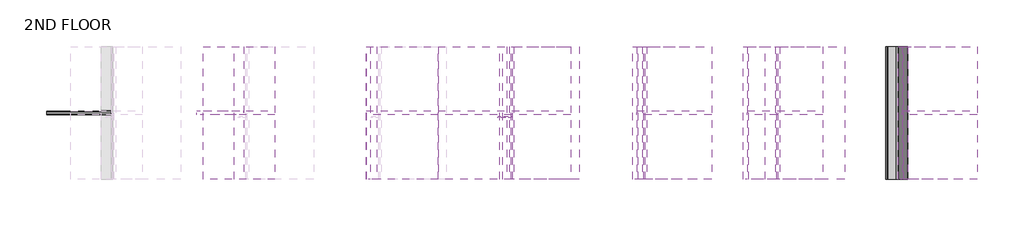
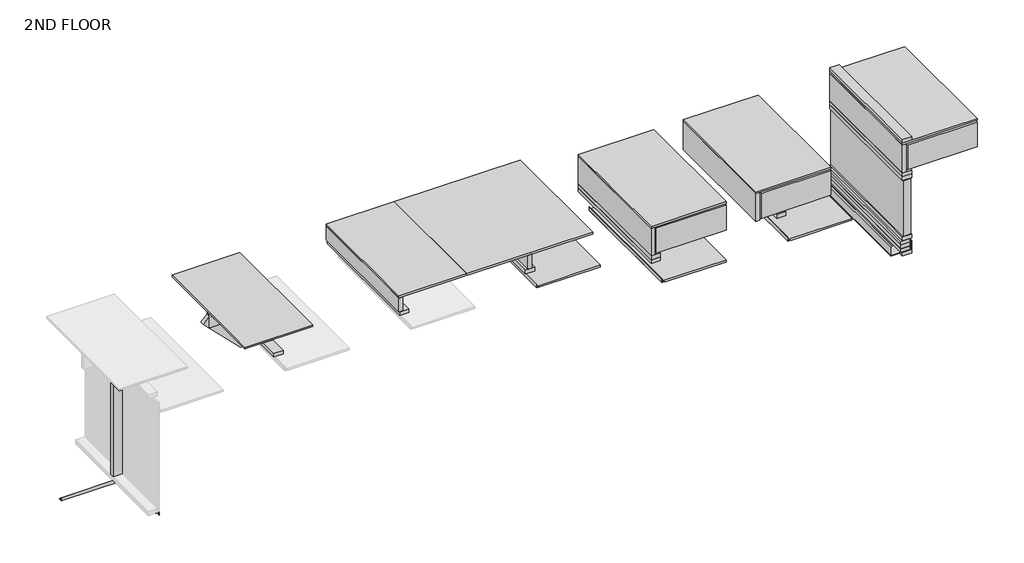
# One storey, part 2 of 2: 51 proxies.
"""IFC4 building model written with IfcOpenShell, lengths in millimetres."""

import ifcopenshell
import ifcopenshell.guid

model = None  # the IFC model being written
_history = None  # IfcOwnerHistory: only IFC2X3 demands one
_inside = {}  # id of a spatial element -> (the spatial element, [elements in it])
_under = {}  # id of a project, library or spatial element -> (it, [spatial elements below it])
_declared = {}  # id of a project -> (the project, [libraries it declares])
_typed = {}  # id of a type object -> (the type object, [elements of that type])
_made_of = {}  # id of a material, layer set ... -> (it, [elements and type objects made of it])


def new_model(schema):
    """Start an empty IFC model of exactly this schema.

    Asked for "IFC4X3", IfcOpenShell would pick the latest addendum, in which some entities
    have other attributes; the version numbers below select the first issue.
    IFC2X3 requires an IfcOwnerHistory on every rooted entity: one is made here for all.
    """
    global model, _history
    if schema == "IFC4X3":
        model = ifcopenshell.file(schema_version=(4, 3, 0, 0))
    else:
        model = ifcopenshell.file(schema=schema)
    _inside.clear()
    _under.clear()
    _declared.clear()
    _typed.clear()
    _made_of.clear()
    _history = None
    if model.schema == "IFC2X3":
        org = make("IfcOrganization", Name="unknown")
        user = make(
            "IfcPersonAndOrganization",
            ThePerson=make("IfcPerson", FamilyName="unknown"),
            TheOrganization=org,
        )
        app = make(
            "IfcApplication",
            ApplicationDeveloper=org,
            Version="unknown",
            ApplicationFullName="unknown",
            ApplicationIdentifier="unknown",
        )
        _history = make(
            "IfcOwnerHistory",
            OwningUser=user,
            OwningApplication=app,
            ChangeAction="ADDED",
            CreationDate=0,
        )
    return model


def make(cls, **values):
    """One entity of the class cls with the attributes given. An attribute that is None is left unset."""
    return model.create_entity(
        cls, **{name: value for name, value in values.items() if value is not None}
    )


def rooted(cls, **values):
    """An entity with a GlobalId (a new one), such as an element, a storey or a relation."""
    return make(cls, GlobalId=ifcopenshell.guid.new(), OwnerHistory=_history, **values)


def si_unit(unit_type, name, prefix=None):
    """IfcSIUnit, for example si_unit("LENGTHUNIT", "METRE", prefix="MILLI")."""
    return make("IfcSIUnit", UnitType=unit_type, Prefix=prefix, Name=name)


def assignment(units):
    """IfcUnitAssignment: the units of a project."""
    return None if units is None else make("IfcUnitAssignment", Units=units)


def point(xyz):
    """IfcCartesianPoint."""
    return None if xyz is None else make("IfcCartesianPoint", Coordinates=xyz)


def direction(xyz):
    """IfcDirection."""
    return None if xyz is None else make("IfcDirection", DirectionRatios=xyz)


def frame(location, z_axis=None, x_axis=None):
    """IfcAxis2Placement3D, a coordinate frame: its origin and axes. An axis left out is left unset."""
    return make(
        "IfcAxis2Placement3D",
        Location=point(location),
        Axis=direction(z_axis),
        RefDirection=direction(x_axis),
    )


def frame_2d(location, x_axis=None):
    """IfcAxis2Placement2D, a coordinate frame in the plane: its origin and x axis."""
    return make(
        "IfcAxis2Placement2D", Location=point(location), RefDirection=direction(x_axis)
    )


def origin():
    """The frame at (0, 0, 0) with its axes left unset."""
    return frame((0.0, 0.0, 0.0))


def place(relative_to, where):
    """IfcLocalPlacement: puts the frame where relative to a parent placement (None: the world)."""
    return make(
        "IfcLocalPlacement", PlacementRelTo=relative_to, RelativePlacement=where
    )


def context(
    kind, dimensions, precision=None, world=None, true_north=None, identifier=None
):
    """IfcGeometricRepresentationContext, for example the 3D "Model" context."""
    return make(
        "IfcGeometricRepresentationContext",
        ContextIdentifier=identifier,
        ContextType=kind,
        CoordinateSpaceDimension=dimensions,
        Precision=precision,
        WorldCoordinateSystem=world,
        TrueNorth=true_north,
    )


def project(units=None, contexts=None):
    """IfcProject with its units and contexts."""
    return rooted(
        "IfcProject",
        Name="project",
        RepresentationContexts=contexts,
        UnitsInContext=assignment(units),
    )


def spatial(cls, under=None, at=None, **own):
    """A site, building, storey or space (cls), placed at a placement, below another one or the project."""
    s = rooted(cls, ObjectPlacement=at, **own)
    if under is not None:
        _under.setdefault(under.id(), (under, []))[1].append(s)
    return s


def polyline(points):
    """IfcPolyline through the points."""
    return make("IfcPolyline", Points=[point(p) for p in points])


def circle_curve(where, radius):
    """IfcCircle in the frame where."""
    return make("IfcCircle", Position=where, Radius=radius)


def trimmed(basis, trim1, trim2, sense, master):
    """IfcTrimmedCurve: the piece of a basis curve between two trims."""
    return make(
        "IfcTrimmedCurve",
        BasisCurve=basis,
        Trim1=trim1,
        Trim2=trim2,
        SenseAgreement=sense,
        MasterRepresentation=master,
    )


def segment(curve, same_sense, transition):
    """IfcCompositeCurveSegment."""
    return make(
        "IfcCompositeCurveSegment",
        Transition=transition,
        SameSense=same_sense,
        ParentCurve=curve,
    )


def composite_curve(segments, self_intersect=None):
    """IfcCompositeCurve: segments joined end to end."""
    return make("IfcCompositeCurve", Segments=segments, SelfIntersect=self_intersect)


def outline(outer, holes=None, kind="AREA"):
    """IfcArbitraryClosedProfileDef: a profile drawn as a closed curve; with holes, ...WithVoids."""
    if holes is None:
        return make("IfcArbitraryClosedProfileDef", ProfileType=kind, OuterCurve=outer)
    return make(
        "IfcArbitraryProfileDefWithVoids",
        ProfileType=kind,
        OuterCurve=outer,
        InnerCurves=holes,
    )


def extrude(swept, where, along, depth):
    """IfcExtrudedAreaSolid: the profile swept, set in the frame where, extruded along a direction by depth."""
    return make(
        "IfcExtrudedAreaSolid",
        SweptArea=swept,
        Position=where,
        ExtrudedDirection=direction(along),
        Depth=depth,
    )


def shape(context_of_items, identifier, shape_type, items):
    """IfcShapeRepresentation: the items that make up one representation, for example the "Body"."""
    return make(
        "IfcShapeRepresentation",
        ContextOfItems=context_of_items,
        RepresentationIdentifier=identifier,
        RepresentationType=shape_type,
        Items=items,
    )


def source(mapping_origin, context_of_items, identifier, shape_type, items):
    """IfcRepresentationMap: a shape defined once, which mapped items show again and again."""
    return make(
        "IfcRepresentationMap",
        MappingOrigin=mapping_origin,
        MappedRepresentation=shape(context_of_items, identifier, shape_type, items),
    )


def transform(
    local_origin,
    x_axis=None,
    y_axis=None,
    z_axis=None,
    scale=None,
    scale2=None,
    scale3=None,
    uniform=True,
):
    """IfcCartesianTransformationOperator3D, or its non-uniform kind. x_axis, y_axis, z_axis: its Axis1, 2, 3."""
    if uniform:
        return make(
            "IfcCartesianTransformationOperator3D",
            Axis1=direction(x_axis),
            Axis2=direction(y_axis),
            LocalOrigin=point(local_origin),
            Scale=scale,
            Axis3=direction(z_axis),
        )
    return make(
        "IfcCartesianTransformationOperator3DnonUniform",
        Axis1=direction(x_axis),
        Axis2=direction(y_axis),
        LocalOrigin=point(local_origin),
        Scale=scale,
        Axis3=direction(z_axis),
        Scale2=scale2,
        Scale3=scale3,
    )


def mapped(mapping_source, mapping_target):
    """IfcMappedItem: shows the shape of a source again, moved by a transform."""
    return make(
        "IfcMappedItem", MappingSource=mapping_source, MappingTarget=mapping_target
    )


def made_of(thing, what):
    """Note that an element or type object is made of a material, layer set ...; save() writes the relation."""
    if what is not None:
        _made_of.setdefault(what.id(), (what, []))[1].append(thing)
    return thing


def element(
    cls,
    number,
    at=None,
    inside=None,
    cuts=None,
    type_object=None,
    material=None,
    context=None,
    identifier="Body",
    shape_type=None,
    held_by="IfcProductDefinitionShape",
    body=None,
    shapes=None,
    **own,
):
    """One element of the class cls, such as IfcWall. Its Tag is "e" and its number.

    at: its placement. inside: the storey or other place that contains it. cuts: it is an
    opening in that element (IfcRelVoidsElement). A single representation is given by context,
    identifier, shape_type and body (its items); several are given by shapes. held_by: the class
    of the entity that holds the representations. save() writes the other relations.
    """
    e = rooted(cls, Tag="e%d" % number, ObjectPlacement=at, **own)
    if body is not None:
        shapes = [shape(context, identifier, shape_type, body)]
    if shapes is not None:
        e.Representation = make(held_by, Representations=shapes)
    if inside is not None:
        _inside.setdefault(inside.id(), (inside, []))[1].append(e)
    if cuts is not None:
        rooted(
            "IfcRelVoidsElement", RelatingBuildingElement=cuts, RelatedOpeningElement=e
        )
    if type_object is not None:
        _typed.setdefault(type_object.id(), (type_object, []))[1].append(e)
    return made_of(e, material)


def aggregate(whole, parts):
    """IfcRelAggregates: a whole, such as a stair, and the parts it consists of."""
    return rooted("IfcRelAggregates", RelatingObject=whole, RelatedObjects=parts)


def save(model, path):
    """Write the relations noted so far, then the file.

    IfcRelAggregates (storeys below a building ...), IfcRelContainedInSpatialStructure (elements
    in a storey), IfcRelDefinesByType, IfcRelAssociatesMaterial and IfcRelDeclares: one each for
    every whole, place, type object, material and project.
    """
    for whole, parts in _under.values():
        aggregate(whole, parts)
    for where, things in _inside.values():
        rooted(
            "IfcRelContainedInSpatialStructure",
            RelatedElements=things,
            RelatingStructure=where,
        )
    for kind, things in _typed.values():
        rooted("IfcRelDefinesByType", RelatedObjects=things, RelatingType=kind)
    for what, things in _made_of.values():
        rooted("IfcRelAssociatesMaterial", RelatedObjects=things, RelatingMaterial=what)
    for by, libraries in _declared.values():
        rooted("IfcRelDeclares", RelatingContext=by, RelatedDefinitions=libraries)
    model.write(path)


def generic_models_10_generic_models_1_ea081297(model_context):
    return source(origin(), model_context, "Body", "SweptSolid", [
        extrude(outline(polyline([(49758.6, 0.0), (49720.5, 0.0), (49720.5, 1219.2), (49758.6, 1219.2), (49758.6, 0.0)])), frame((0.0, 0.0, 5507.83125), z_axis=(0.0, 0.0, 1.0), x_axis=(1.0, 0.0, 0.0)), (0.0, 0.0, 1.0), 139.7),
    ])


def generic_models_102_generic_models_1_8a2dd616(model_context):
    return source(origin(), model_context, "Body", "SweptSolid", [
        extrude(outline(composite_curve([segment(polyline([(4498.578125, 52222.4), (4510.823229, 52207.8068534), (4508.6950617, 52206.021109), (4497.282664, 52219.621875), (4414.3677682, 52219.621875)]), True, "CONTINUOUS"), segment(trimmed(circle_curve(frame_2d((4414.4412941, 52217.6381931)), 1.9850441), [point((4414.3677682, 52219.621875))], [point((4412.45625, 52217.6381931))], True, "CARTESIAN"), True, "CONTINUOUS"), segment(polyline([(4412.45625, 52217.6381931), (4412.45625, 52023.9610661)]), True, "CONTINUOUS"), segment(trimmed(circle_curve(frame_2d((4414.4419899, 52023.9610661)), 1.9857399), [point((4412.45625, 52023.9610661))], [point((4414.3365981, 52021.978125))], True, "CARTESIAN"), True, "CONTINUOUS"), segment(polyline([(4414.3365981, 52021.978125), (4497.282664, 52021.978125), (4508.718285, 52035.6065673), (4510.8464522, 52033.820823), (4498.578125, 52019.2), (4414.440625, 52019.2)]), True, "CONTINUOUS"), segment(trimmed(circle_curve(frame_2d((4414.440625, 52023.9625)), 4.7625), [point((4414.440625, 52019.2))], [point((4409.678125, 52023.9625))], False, "CARTESIAN"), True, "CONTINUOUS"), segment(polyline([(4409.678125, 52023.9625), (4409.678125, 52217.6375)]), True, "CONTINUOUS"), segment(trimmed(circle_curve(frame_2d((4414.440625, 52217.6375)), 4.7625), [point((4409.678125, 52217.6375))], [point((4414.440625, 52222.4))], False, "CARTESIAN"), True, "CONTINUOUS"), segment(polyline([(4414.440625, 52222.4), (4498.578125, 52222.4)]), True, "CONTINUOUS")], self_intersect=False)), frame((0.0, 0.0, 0.0), z_axis=(0.0, 1.0, 0.0), x_axis=(0.0, 0.0, 1.0)), (0.0, 0.0, 1.0), 1219.2),
    ])


def generic_models_103_generic_models_1_250a6a11(model_context):
    return source(origin(), model_context, "Body", "SweptSolid", [
        extrude(outline(polyline([(49784.0, 0.0), (49695.1, 0.0), (49695.1, 1219.2), (49784.0, 1219.2), (49784.0, 0.0)])), frame((0.0, 0.0, 5264.15), z_axis=(0.0, 0.0, 1.0), x_axis=(1.0, 0.0, 0.0)), (0.0, 0.0, 1.0), 38.1),
    ])


def generic_models_104_generic_models_1_af33e5d9(model_context):
    return source(origin(), model_context, "Body", "SweptSolid", [
        extrude(outline(polyline([(52206.021109, 0.0), (52117.121109, 0.0), (52117.121109, 1219.2), (52206.021109, 1219.2), (52206.021109, 0.0)])), frame((0.0, 0.0, 4412.45625), z_axis=(0.0, 0.0, 1.0), x_axis=(1.0, 0.0, 0.0)), (0.0, 0.0, 1.0), 38.1),
    ])


def generic_models_108_generic_models_1_496acf5e(model_context):
    return source(origin(), model_context, "Body", "SweptSolid", [
        extrude(outline(polyline([(52216.05, 1219.2), (52216.05, 0.0), (52139.85, 0.0), (52139.85, 1219.2), (52216.05, 1219.2)])), frame((0.0, 0.0, 4570.4125), z_axis=(0.0, 0.0, 1.0), x_axis=(1.0, 0.0, 0.0)), (0.0, 0.0, 1.0), 565.15),
    ])


def generic_models_109_generic_models_1_8619d77b(model_context):
    return source(origin(), model_context, "Body", "SweptSolid", [
        extrude(outline(polyline([(51003.2, 0.0), (50914.3, 0.0), (50914.3, 1219.2), (51003.2, 1219.2), (51003.2, 0.0)])), frame((0.0, 0.0, 5184.378125), z_axis=(0.0, 0.0, 1.0), x_axis=(1.0, 0.0, 0.0)), (0.0, 0.0, 1.0), 38.1),
    ])


def generic_models_110_generic_models_1_6bdce9b6(model_context):
    return source(origin(), model_context, "Body", "SweptSolid", [
        extrude(outline(polyline([(51642.1451407, 1219.2), (51642.1451407, 0.0), (50914.3, 0.0), (50914.3, 1219.2), (51642.1451407, 1219.2)])), frame((0.0, 0.0, 5508.228125), z_axis=(0.0, 0.0, 1.0), x_axis=(1.0, 0.0, 0.0)), (0.0, 0.0, 1.0), 19.05),
    ])


def generic_models_112_generic_models_65_d168d7b0(model_context):
    return source(origin(), model_context, "Body", "SweptSolid", [
        extrude(outline(polyline([(50952.4, 592.1375), (50952.4, 630.2375), (51642.1451407, 630.2375), (51642.1451407, 592.1375), (50952.4, 592.1375)])), frame((0.0, 0.0, 5222.478125), z_axis=(0.0, 0.0, 1.0), x_axis=(1.0, 0.0, 0.0)), (0.0, 0.0, 1.0), 285.75),
    ])


def generic_models_113_generic_models_1_101608ab(model_context):
    return source(origin(), model_context, "Body", "SweptSolid", [
        extrude(outline(polyline([(52171.6, 0.0), (52133.5, 0.0), (52133.5, 1219.2), (52171.6, 1219.2), (52171.6, 0.0)])), frame((0.0, 0.0, 5222.478125), z_axis=(0.0, 0.0, 1.0), x_axis=(1.0, 0.0, 0.0)), (0.0, 0.0, 1.0), 285.75),
    ])


def generic_models_114_generic_models_1_a6fb1c2c(model_context):
    return source(origin(), model_context, "Body", "SweptSolid", [
        extrude(outline(polyline([(51642.1451407, 1219.2), (51642.1451407, 0.0), (50965.9242022, 0.0), (50965.9242022, 1219.2), (51642.1451407, 1219.2)])), frame((0.0, 0.0, 5237.6235034), z_axis=(0.0, 0.0, 1.0), x_axis=(1.0, 0.0, 0.0)), (0.0, 0.0, 1.0), 254.0),
    ])


def generic_models_12_generic_models_46_b8a9a4e8(model_context):
    return source(origin(), model_context, "Body", "SweptSolid", [
        extrude(outline(polyline([(49757.8505137, 0.0), (49721.1284797, 0.0), (49721.1284797, 1219.2), (49757.8505137, 1219.2), (49757.8505137, 0.0)])), frame((0.0, 0.0, 5505.7509163), z_axis=(0.0, 0.0, 1.0), x_axis=(1.0, 0.0, 0.0)), (0.0, 0.0, 1.0), 1.5875),
    ])


def generic_models_13_generic_models_65_9e643fb9(model_context):
    return source(origin(), model_context, "Body", "SweptSolid", [
        extrude(outline(polyline([(49128.3625, 592.1375), (49128.3625, 630.2375), (50347.5625, 630.2375), (50347.5625, 592.1375), (49128.3625, 592.1375)])), frame((0.0, 0.0, 5507.83125), z_axis=(0.0, 0.0, 1.0), x_axis=(1.0, 0.0, 0.0)), (0.0, 0.0, 1.0), 139.7),
    ])


def generic_models_14_generic_models_1_e8c90d4c(model_context):
    return source(origin(), model_context, "Body", "SweptSolid", [
        extrude(outline(polyline([(2277.1204978, 49799.875), (2239.0204978, 49799.875), (2239.0204978, 49825.275), (2240.6079978, 49825.275), (2240.6079978, 49801.4625), (2277.1204978, 49801.4625), (2277.1204978, 49799.875)])), frame((0.0, 0.0, 0.0), z_axis=(0.0, 1.0, 0.0), x_axis=(0.0, 0.0, 1.0)), (0.0, 0.0, 1.0), 1219.2),
    ])


def generic_models_22_generic_models_1_e5767157(model_context):
    return source(origin(), model_context, "Body", "SweptSolid", [
        extrude(outline(polyline([(2409.6091, 49800.66875), (2409.6091, 49799.875), (2407.0592364, 49799.875), (2405.4618473, 49749.075), (2404.6631527, 49749.075), (2403.0657636, 49799.875), (2400.5159, 49799.875), (2400.5159, 49800.66875), (2409.6091, 49800.66875)])), frame((0.0, 565.15, 0.0), z_axis=(0.0, 1.0, 0.0), x_axis=(0.0, 0.0, 1.0)), (0.0, 0.0, 1.0), 12.7),
    ])


def generic_models_228_generic_models_1_053e8907(model_context):
    return source(origin(), model_context, "Body", "SweptSolid", [
        extrude(outline(composite_curve([segment(polyline([(592.1375, 4235.45), (592.1375, 4267.2)]), True, "CONTINUOUS"), segment(trimmed(circle_curve(frame_2d((592.1375, 4264.025)), 3.175), [point((592.1375, 4267.2))], [point((595.3125, 4264.025))], False, "CARTESIAN"), True, "CONTINUOUS"), segment(polyline([(595.3125, 4264.025), (595.3125, 4240.2125)]), True, "CONTINUOUS"), segment(trimmed(circle_curve(frame_2d((596.9, 4240.2125)), 1.5875), [point((595.3125, 4240.2125))], [point((596.9, 4238.625))], True, "CARTESIAN"), True, "CONTINUOUS"), segment(polyline([(596.9, 4238.625), (620.7125, 4238.625)]), True, "CONTINUOUS"), segment(trimmed(circle_curve(frame_2d((620.7125, 4235.45)), 3.175), [point((620.7125, 4238.625))], [point((623.8875, 4235.45))], False, "CARTESIAN"), True, "CONTINUOUS"), segment(polyline([(623.8875, 4235.45), (592.1375, 4235.45)]), True, "CONTINUOUS")], self_intersect=False)), frame((46753.4625, 0.0, 0.0), z_axis=(1.0, 0.0, 0.0), x_axis=(0.0, 1.0, 0.0)), (0.0, 0.0, 1.0), 609.6),
    ])


def generic_models_233_generic_models_1_ae5bae41(model_context):
    return source(origin(), model_context, "Body", "SweptSolid", [
        extrude(outline(polyline([(48564.8, 0.0), (48475.9, 0.0), (48475.9, 1219.2), (48564.8, 1219.2), (48564.8, 0.0)])), frame((0.0, 0.0, 5467.35), z_axis=(0.0, 0.0, 1.0), x_axis=(1.0, 0.0, 0.0)), (0.0, 0.0, 1.0), 38.1),
    ])


def generic_models_236_generic_models_1_f8917e71(model_context):
    return source(origin(), model_context, "Body", "SweptSolid", [
        extrude(outline(polyline([(48507.65, 0.0), (48469.55, 0.0), (48469.55, 1219.2), (48507.65, 1219.2), (48507.65, 0.0)])), frame((0.0, 0.0, 5507.83125), z_axis=(0.0, 0.0, 1.0), x_axis=(1.0, 0.0, 0.0)), (0.0, 0.0, 1.0), 139.7),
    ])


def generic_models_237_generic_models_65_1df05f16(model_context):
    return source(origin(), model_context, "Body", "SweptSolid", [
        extrude(outline(polyline([(48469.55, 592.1375), (48469.55, 630.2375), (49128.3625, 630.2375), (49128.3625, 592.1375), (48469.55, 592.1375)])), frame((0.0, 0.0, 5507.83125), z_axis=(0.0, 0.0, 1.0), x_axis=(1.0, 0.0, 0.0)), (0.0, 0.0, 1.0), 139.7),
    ])


def generic_models_240_generic_models_1_611786cf(model_context):
    return source(origin(), model_context, "Body", "SweptSolid", [
        extrude(outline(polyline([(49128.3625, 1219.2), (49128.3625, 0.0), (48469.55, 0.0), (48469.55, 1219.2), (49128.3625, 1219.2)])), frame((0.0, 0.0, 5649.9125), z_axis=(0.0, 0.0, 1.0), x_axis=(1.0, 0.0, 0.0)), (0.0, 0.0, 1.0), 19.05),
    ])


def generic_models_246_generic_models_1_33f707d8(model_context):
    return source(origin(), model_context, "Body", "SweptSolid", [
        extrude(outline(composite_curve([segment(polyline([(4267.2, 47363.0625), (4267.2, 47331.3125)]), True, "CONTINUOUS"), segment(trimmed(circle_curve(frame_2d((4267.2, 47334.4875)), 3.175), [point((4267.2, 47331.3125))], [point((4264.025, 47334.4875))], False, "CARTESIAN"), True, "CONTINUOUS"), segment(polyline([(4264.025, 47334.4875), (4264.025, 47358.3)]), True, "CONTINUOUS"), segment(trimmed(circle_curve(frame_2d((4262.4375, 47358.3)), 1.5875), [point((4264.025, 47358.3))], [point((4262.4375, 47359.8875))], True, "CARTESIAN"), True, "CONTINUOUS"), segment(polyline([(4262.4375, 47359.8875), (4238.625, 47359.8875)]), True, "CONTINUOUS"), segment(trimmed(circle_curve(frame_2d((4238.625, 47363.0625)), 3.175), [point((4238.625, 47359.8875))], [point((4235.45, 47363.0625))], False, "CARTESIAN"), True, "CONTINUOUS"), segment(polyline([(4235.45, 47363.0625), (4267.2, 47363.0625)]), True, "CONTINUOUS")], self_intersect=False)), frame((0.0, 0.0, 0.0), z_axis=(0.0, 1.0, 0.0), x_axis=(0.0, 0.0, 1.0)), (0.0, 0.0, 1.0), 1219.2),
    ])


def generic_models_248_generic_models_65_f6c484d7(model_context):
    return source(origin(), model_context, "Body", "SweptSolid", [
        extrude(outline(polyline([(47345.6, 592.1375), (47256.7, 592.1375), (47256.7, 630.2375), (47345.6, 630.2375), (47345.6, 592.1375)])), frame((0.0, 0.0, 4305.3), z_axis=(0.0, 0.0, 1.0), x_axis=(1.0, 0.0, 0.0)), (0.0, 0.0, 1.0), 1162.05),
    ])


def generic_models_267_generic_models_65_11354230(model_context):
    return source(origin(), model_context, "Body", "SweptSolid", [
        extrude(outline(polyline([(0.0, -38.1), (0.0, 0.0), (514.35, 0.0), (514.35, -38.1), (0.0, -38.1)])), frame((47276.4596037, 592.1375, 5202.484661), z_axis=(0.7071067811865633, 0.0, 0.7071067811865317), x_axis=(-0.7071067811865317, 0.0, 0.7071067811865633)), (0.0, 0.0, 1.0), 88.9),
    ])


def generic_models_29_generic_models_1_59087225(model_context):
    return source(origin(), model_context, "Body", "SweptSolid", [
        extrude(outline(polyline([(50347.5625, 1219.2), (50347.5625, 0.0), (49128.3625, 0.0), (49128.3625, 1219.2), (50347.5625, 1219.2)])), frame((0.0, 0.0, 5647.53125), z_axis=(0.0, 0.0, 1.0), x_axis=(1.0, 0.0, 0.0)), (0.0, 0.0, 1.0), 19.05),
    ])


def generic_models_226_generic_models_1_7dc37832(model_context):
    return source(origin(), model_context, "Body", "SweptSolid", [
        extrude(outline(polyline([(5263.35625, 49733.4159), (5263.35625, 49742.5091), (5264.15, 49742.5091), (5264.15, 49739.9592364), (5314.95, 49738.3618473), (5314.95, 49737.5631527), (5264.15, 49735.9657636), (5264.15, 49733.4159), (5263.35625, 49733.4159)])), frame((0.0, 565.15, 0.0), z_axis=(0.0, 1.0, 0.0), x_axis=(0.0, 0.0, 1.0)), (0.0, 0.0, 1.0), 12.7),
    ])


def generic_models_37_generic_models_1_916dd7c6(model_context):
    return source(origin(), model_context, "Body", "SweptSolid", [
        extrude(outline(polyline([(2409.6091, 49675.25625), (2400.5159, 49675.25625), (2400.5159, 49676.05), (2403.0657636, 49676.05), (2404.6631527, 49726.85), (2405.4618473, 49726.85), (2407.0592364, 49676.05), (2409.6091, 49676.05), (2409.6091, 49675.25625)])), frame((0.0, 565.15, 0.0), z_axis=(0.0, 1.0, 0.0), x_axis=(0.0, 0.0, 1.0)), (0.0, 0.0, 1.0), 12.7),
    ])


def generic_models_202_generic_models_1_0ad20a8b(model_context):
    return source(origin(), model_context, "Body", "SweptSolid", [
        extrude(outline(polyline([(2253.330428, 49813.3451407), (2242.217928, 49813.3451407), (2242.217928, 49826.0451407), (2234.280428, 49828.9341545), (2234.280428, 50422.9451407), (2253.330428, 50422.9451407), (2253.330428, 49813.3451407)])), frame((0.0, 0.0, 0.0), z_axis=(0.0, 1.0, 0.0), x_axis=(0.0, 0.0, 1.0)), (0.0, 0.0, 1.0), 1219.2),
    ])


def generic_models_71_generic_models_1_508a995f(model_context):
    return source(origin(), model_context, "Body", "SweptSolid", [
        extrude(outline(polyline([(50952.4, 0.0), (50914.3, 0.0), (50914.3, 1219.2), (50952.4, 1219.2), (50952.4, 0.0)])), frame((0.0, 0.0, 5222.478125), z_axis=(0.0, 0.0, 1.0), x_axis=(1.0, 0.0, 0.0)), (0.0, 0.0, 1.0), 285.75),
    ])


def generic_models_87_generic_models_1_55a64953(model_context):
    return source(origin(), model_context, "Body", "SweptSolid", [
        extrude(outline(polyline([(51968.4, 0.0), (51930.3, 0.0), (51930.3, 1219.2), (51968.4, 1219.2), (51968.4, 0.0)])), frame((0.0, 0.0, 5222.478125), z_axis=(0.0, 0.0, 1.0), x_axis=(1.0, 0.0, 0.0)), (0.0, 0.0, 1.0), 285.75),
    ])


model = new_model("IFC4")

# Units and contexts
model_context = context("Model", 3, world=origin())
ifc_project = project(units=[si_unit("LENGTHUNIT", "METRE", prefix="MILLI")], contexts=[model_context])

# Site, building, storey
site = spatial("IfcSite", under=ifc_project)
building = spatial("IfcBuilding", under=site)
storey = spatial("IfcBuildingStorey", under=building, Name="2ND FLOOR", Elevation=3657.6)

# Proxies
placement = place(None, origin())
generic_models_10_generic_models_1_shape = generic_models_10_generic_models_1_ea081297(model_context)
element("IfcBuildingElementProxy", 1, Name="Generic Models 10 : Generic Models 1", ObjectType="Generic Models 10 : Generic Models 1", at=placement, inside=storey, context=model_context, shape_type="MappedRepresentation", body=[
    mapped(generic_models_10_generic_models_1_shape, transform((0.0, 0.0, 0.0), x_axis=(1.0, 0.0, 0.0), y_axis=(0.0, 1.0, 0.0), z_axis=(0.0, 0.0, 1.0))),
])
generic_models_102_generic_models_1_shape = generic_models_102_generic_models_1_8a2dd616(model_context)
element("IfcBuildingElementProxy", 2, Name="Generic Models 102 : Generic Models 1", ObjectType="Generic Models 102 : Generic Models 1", at=placement, inside=storey, context=model_context, shape_type="MappedRepresentation", body=[
    mapped(generic_models_102_generic_models_1_shape, transform((1219.2, 0.0, 0.0), x_axis=(1.0, 0.0, 0.0), y_axis=(0.0, 1.0, 0.0), z_axis=(0.0, 0.0, 1.0))),
])
generic_models_103_generic_models_1_shape = generic_models_103_generic_models_1_250a6a11(model_context)
element("IfcBuildingElementProxy", 3, Name="Generic Models 103 : Generic Models 1", ObjectType="Generic Models 103 : Generic Models 1", at=placement, inside=storey, context=model_context, shape_type="MappedRepresentation", body=[
    mapped(generic_models_103_generic_models_1_shape, transform((3657.6, 0.0, -892.571875), x_axis=(1.0, 0.0, 0.0), y_axis=(0.0, 1.0, 0.0), z_axis=(0.0, 0.0, 1.0))),
])
generic_models_104_generic_models_1_shape = generic_models_104_generic_models_1_af33e5d9(model_context)
element("IfcBuildingElementProxy", 4, Name="Generic Models 104 : Generic Models 1", ObjectType="Generic Models 104 : Generic Models 1", at=placement, inside=storey, context=model_context, shape_type="MappedRepresentation", body=[
    mapped(generic_models_104_generic_models_1_shape, transform((1219.2, 0.0, 0.0), x_axis=(1.0, 0.0, 0.0), y_axis=(0.0, 1.0, 0.0), z_axis=(0.0, 0.0, 1.0))),
])
element("IfcBuildingElementProxy", 5, Name="Generic Models 105 : Generic Models 1", ObjectType="Generic Models 105 : Generic Models 1", at=placement, inside=storey, context=model_context, shape_type="MappedRepresentation", body=[
    mapped(generic_models_103_generic_models_1_shape, transform((3641.221109, 0.0, -813.59375), x_axis=(1.0, 0.0, 0.0), y_axis=(0.0, 1.0, 0.0), z_axis=(0.0, 0.0, 1.0))),
])
element("IfcBuildingElementProxy", 6, Name="Generic Models 106 : Generic Models 1", ObjectType="Generic Models 106 : Generic Models 1", at=placement, inside=storey, context=model_context, shape_type="MappedRepresentation", body=[
    mapped(generic_models_103_generic_models_1_shape, transform((3641.221109, 0.0, -775.49375), x_axis=(1.0, 0.0, 0.0), y_axis=(0.0, 1.0, 0.0), z_axis=(0.0, 0.0, 1.0))),
])
element("IfcBuildingElementProxy", 7, Name="Generic Models 107 : Generic Models 1", ObjectType="Generic Models 107 : Generic Models 1", at=placement, inside=storey, context=model_context, shape_type="MappedRepresentation", body=[
    mapped(generic_models_103_generic_models_1_shape, transform((3657.6, 0.0, -737.39375), x_axis=(1.0, 0.0, 0.0), y_axis=(0.0, 1.0, 0.0), z_axis=(0.0, 0.0, 1.0))),
])
generic_models_108_generic_models_1_shape = generic_models_108_generic_models_1_496acf5e(model_context)
element("IfcBuildingElementProxy", 8, Name="Generic Models 108 : Generic Models 1", ObjectType="Generic Models 108 : Generic Models 1", at=placement, inside=storey, context=model_context, shape_type="MappedRepresentation", body=[
    mapped(generic_models_108_generic_models_1_shape, transform((1219.2, 0.0, 0.0), x_axis=(1.0, 0.0, 0.0), y_axis=(0.0, 1.0, 0.0), z_axis=(0.0, 0.0, 1.0))),
])
generic_models_109_generic_models_1_shape = generic_models_109_generic_models_1_8619d77b(model_context)
element("IfcBuildingElementProxy", 9, Name="Generic Models 109 : Generic Models 1", ObjectType="Generic Models 109 : Generic Models 1", at=placement, inside=storey, context=model_context, shape_type="MappedRepresentation", body=[
    mapped(generic_models_109_generic_models_1_shape, transform((2438.4, 0.0, 0.0), x_axis=(1.0, 0.0, 0.0), y_axis=(0.0, 1.0, 0.0), z_axis=(0.0, 0.0, 1.0))),
])
generic_models_110_generic_models_1_shape = generic_models_110_generic_models_1_6bdce9b6(model_context)
element("IfcBuildingElementProxy", 10, Name="Generic Models 110 : Generic Models 1", ObjectType="Generic Models 110 : Generic Models 1", at=placement, inside=storey, context=model_context, shape_type="MappedRepresentation", body=[
    mapped(generic_models_110_generic_models_1_shape, transform((2438.4, 0.0, 0.0), x_axis=(1.0, 0.0, 0.0), y_axis=(0.0, 1.0, 0.0), z_axis=(0.0, 0.0, 1.0))),
])
element("IfcBuildingElementProxy", 11, Name="Generic Models 111 : Generic Models 1", ObjectType="Generic Models 111 : Generic Models 1", at=placement, inside=storey, context=model_context, shape_type="MappedRepresentation", body=[
    mapped(generic_models_109_generic_models_1_shape, transform((2438.4, 0.0, -38.1), x_axis=(1.0, 0.0, 0.0), y_axis=(0.0, 1.0, 0.0), z_axis=(0.0, 0.0, 1.0))),
])
generic_models_112_generic_models_65_shape = generic_models_112_generic_models_65_d168d7b0(model_context)
element("IfcBuildingElementProxy", 12, Name="Generic Models 112 : Generic Models 65", ObjectType="Generic Models 112 : Generic Models 65", at=placement, inside=storey, context=model_context, shape_type="MappedRepresentation", body=[
    mapped(generic_models_112_generic_models_65_shape, transform((2438.4, 0.0, 0.0), x_axis=(1.0, 0.0, 0.0), y_axis=(0.0, 1.0, 0.0), z_axis=(0.0, 0.0, 1.0))),
])
generic_models_113_generic_models_1_shape = generic_models_113_generic_models_1_101608ab(model_context)
element("IfcBuildingElementProxy", 13, Name="Generic Models 113 : Generic Models 1", ObjectType="Generic Models 113 : Generic Models 1", at=placement, inside=storey, context=model_context, shape_type="MappedRepresentation", body=[
    mapped(generic_models_113_generic_models_1_shape, transform((1219.2, 0.0, 0.0), x_axis=(1.0, 0.0, 0.0), y_axis=(0.0, 1.0, 0.0), z_axis=(0.0, 0.0, 1.0))),
])
generic_models_114_generic_models_1_shape = generic_models_114_generic_models_1_a6fb1c2c(model_context)
element("IfcBuildingElementProxy", 14, Name="Generic Models 114 : Generic Models 1", ObjectType="Generic Models 114 : Generic Models 1", at=placement, inside=storey, context=model_context, shape_type="MappedRepresentation", body=[
    mapped(generic_models_114_generic_models_1_shape, transform((2438.4, 0.0, 0.0), x_axis=(1.0, 0.0, 0.0), y_axis=(0.0, 1.0, 0.0), z_axis=(0.0, 0.0, 1.0))),
])
element("IfcBuildingElementProxy", 15, Name="Generic Models 115 : Generic Models 1", ObjectType="Generic Models 115 : Generic Models 1", at=placement, inside=storey, context=model_context, shape_type="MappedRepresentation", body=[
    mapped(generic_models_109_generic_models_1_shape, transform((2438.4, 0.0, 342.9), x_axis=(1.0, 0.0, 0.0), y_axis=(0.0, 1.0, 0.0), z_axis=(0.0, 0.0, 1.0))),
])
generic_models_12_generic_models_46_shape = generic_models_12_generic_models_46_b8a9a4e8(model_context)
element("IfcBuildingElementProxy", 16, Name="Generic Models 12 : Generic Models 46", ObjectType="Generic Models 12 : Generic Models 46", at=placement, inside=storey, context=model_context, shape_type="MappedRepresentation", body=[
    mapped(generic_models_12_generic_models_46_shape, transform((0.0, 0.0, 0.0), x_axis=(1.0, 0.0, 0.0), y_axis=(0.0, 1.0, 0.0), z_axis=(0.0, 0.0, 1.0))),
])
generic_models_13_generic_models_65_shape = generic_models_13_generic_models_65_9e643fb9(model_context)
element("IfcBuildingElementProxy", 17, Name="Generic Models 13 : Generic Models 65", ObjectType="Generic Models 13 : Generic Models 65", at=placement, inside=storey, context=model_context, shape_type="MappedRepresentation", body=[
    mapped(generic_models_13_generic_models_65_shape, transform((0.0, 0.0, 0.0), x_axis=(1.0, 0.0, 0.0), y_axis=(0.0, 1.0, 0.0), z_axis=(0.0, 0.0, 1.0))),
])
generic_models_14_generic_models_1_shape = generic_models_14_generic_models_1_e8c90d4c(model_context)
element("IfcBuildingElementProxy", 18, Name="Generic Models 14 : Generic Models 1", ObjectType="Generic Models 14 : Generic Models 1", at=placement, inside=storey, context=model_context, shape_type="MappedRepresentation", body=[
    mapped(generic_models_14_generic_models_1_shape, transform((0.0, 0.0, 3050.778125), x_axis=(1.0, 0.0, 0.0), y_axis=(0.0, 1.0, 0.0), z_axis=(0.0, 0.0, 1.0))),
])
generic_models_22_generic_models_1_shape = generic_models_22_generic_models_1_e5767157(model_context)
element("IfcBuildingElementProxy", 19, Name="Generic Models 22 : Generic Models 1", ObjectType="Generic Models 22 : Generic Models 1", at=placement, inside=storey, context=model_context, shape_type="MappedRepresentation", body=[
    mapped(generic_models_22_generic_models_1_shape, transform((0.0, 0.0, 3081.3375), x_axis=(1.0, 0.0, 0.0), y_axis=(0.0, 1.0, 0.0), z_axis=(0.0, 0.0, 1.0))),
])
generic_models_228_generic_models_1_shape = generic_models_228_generic_models_1_053e8907(model_context)
element("IfcBuildingElementProxy", 20, Name="Generic Models 228 : Generic Models 1", ObjectType="Generic Models 228 : Generic Models 1", at=placement, inside=storey, context=model_context, shape_type="MappedRepresentation", body=[
    mapped(generic_models_228_generic_models_1_shape, transform((-1219.2, 0.0, 0.0), x_axis=(1.0, 0.0, 0.0), y_axis=(0.0, 1.0, 0.0), z_axis=(0.0, 0.0, 1.0))),
])
generic_models_233_generic_models_1_shape = generic_models_233_generic_models_1_ae5bae41(model_context)
element("IfcBuildingElementProxy", 21, Name="Generic Models 233 : Generic Models 1", ObjectType="Generic Models 233 : Generic Models 1", at=placement, inside=storey, context=model_context, shape_type="MappedRepresentation", body=[
    mapped(generic_models_233_generic_models_1_shape, transform((0.0, 0.0, 0.0), x_axis=(1.0, 0.0, 0.0), y_axis=(0.0, 1.0, 0.0), z_axis=(0.0, 0.0, 1.0))),
])
generic_models_236_generic_models_1_shape = generic_models_236_generic_models_1_f8917e71(model_context)
element("IfcBuildingElementProxy", 22, Name="Generic Models 236 : Generic Models 1", ObjectType="Generic Models 236 : Generic Models 1", at=placement, inside=storey, context=model_context, shape_type="MappedRepresentation", body=[
    mapped(generic_models_236_generic_models_1_shape, transform((0.0, 0.0, 0.0), x_axis=(1.0, 0.0, 0.0), y_axis=(0.0, 1.0, 0.0), z_axis=(0.0, 0.0, 1.0))),
])
generic_models_237_generic_models_65_shape = generic_models_237_generic_models_65_1df05f16(model_context)
element("IfcBuildingElementProxy", 23, Name="Generic Models 237 : Generic Models 65", ObjectType="Generic Models 237 : Generic Models 65", at=placement, inside=storey, context=model_context, shape_type="MappedRepresentation", body=[
    mapped(generic_models_237_generic_models_65_shape, transform((0.0, 0.0, 0.0), x_axis=(1.0, 0.0, 0.0), y_axis=(0.0, 1.0, 0.0), z_axis=(0.0, 0.0, 1.0))),
])
generic_models_240_generic_models_1_shape = generic_models_240_generic_models_1_611786cf(model_context)
element("IfcBuildingElementProxy", 24, Name="Generic Models 240 : Generic Models 1", ObjectType="Generic Models 240 : Generic Models 1", at=placement, inside=storey, context=model_context, shape_type="MappedRepresentation", body=[
    mapped(generic_models_240_generic_models_1_shape, transform((0.0, 0.0, 0.0), x_axis=(1.0, 0.0, 0.0), y_axis=(0.0, 1.0, 0.0), z_axis=(0.0, 0.0, 1.0))),
])
generic_models_246_generic_models_1_shape = generic_models_246_generic_models_1_33f707d8(model_context)
element("IfcBuildingElementProxy", 25, Name="Generic Models 246 : Generic Models 1", ObjectType="Generic Models 246 : Generic Models 1", at=placement, inside=storey, context=model_context, shape_type="MappedRepresentation", body=[
    mapped(generic_models_246_generic_models_1_shape, transform((-1219.2, 0.0, 0.0), x_axis=(1.0, 0.0, 0.0), y_axis=(0.0, 1.0, 0.0), z_axis=(0.0, 0.0, 1.0))),
])
generic_models_248_generic_models_65_shape = generic_models_248_generic_models_65_f6c484d7(model_context)
element("IfcBuildingElementProxy", 26, Name="Generic Models 248 : Generic Models 65", ObjectType="Generic Models 248 : Generic Models 65", at=placement, inside=storey, context=model_context, shape_type="MappedRepresentation", body=[
    mapped(generic_models_248_generic_models_65_shape, transform((-1219.2, 0.0, 0.0), x_axis=(1.0, 0.0, 0.0), y_axis=(0.0, 1.0, 0.0), z_axis=(0.0, 0.0, 1.0))),
])
element("IfcBuildingElementProxy", 27, Name="Generic Models 25 : Generic Models 46", ObjectType="Generic Models 25 : Generic Models 46", at=placement, inside=storey, context=model_context, shape_type="MappedRepresentation", body=[
    mapped(generic_models_12_generic_models_46_shape, transform((0.0, 0.0, 142.08125), x_axis=(1.0, 0.0, 0.0), y_axis=(0.0, 1.0, 0.0), z_axis=(0.0, 0.0, 1.0))),
])
element("IfcBuildingElementProxy", 28, Name="Generic Models 261 : Generic Models 1", ObjectType="Generic Models 261 : Generic Models 1", at=placement, inside=storey, context=model_context, shape_type="MappedRepresentation", body=[
    mapped(generic_models_233_generic_models_1_shape, transform((-1219.2, 0.0, 0.0), x_axis=(1.0, 0.0, 0.0), y_axis=(0.0, 1.0, 0.0), z_axis=(0.0, 0.0, 1.0))),
])
element("IfcBuildingElementProxy", 29, Name="Generic Models 264 : Generic Models 65", ObjectType="Generic Models 264 : Generic Models 65", at=placement, inside=storey, context=model_context, shape_type="MappedRepresentation", body=[
    mapped(generic_models_237_generic_models_65_shape, transform((-1497.80625, 0.0, 0.0), x_axis=(1.0, 0.0, 0.0), y_axis=(0.0, 1.0, 0.0), z_axis=(0.0, 0.0, 1.0))),
])
element("IfcBuildingElementProxy", 30, Name="Generic Models 266 : Generic Models 1", ObjectType="Generic Models 266 : Generic Models 1", at=placement, inside=storey, context=model_context, shape_type="MappedRepresentation", body=[
    mapped(generic_models_240_generic_models_1_shape, transform((-1497.80625, 0.0, 0.0), x_axis=(1.0, 0.0, 0.0), y_axis=(0.0, 1.0, 0.0), z_axis=(0.0, 0.0, 1.0))),
])
generic_models_267_generic_models_65_shape = generic_models_267_generic_models_65_11354230(model_context)
element("IfcBuildingElementProxy", 31, Name="Generic Models 267 : Generic Models 65", ObjectType="Generic Models 267 : Generic Models 65", at=placement, inside=storey, context=model_context, shape_type="MappedRepresentation", body=[
    mapped(generic_models_267_generic_models_65_shape, transform((0.0, 0.0, 0.0), x_axis=(1.0, 0.0, 0.0), y_axis=(0.0, 1.0, 0.0), z_axis=(0.0, 0.0, 1.0))),
])
generic_models_29_generic_models_1_shape = generic_models_29_generic_models_1_59087225(model_context)
element("IfcBuildingElementProxy", 32, Name="Generic Models 29 : Generic Models 1", ObjectType="Generic Models 29 : Generic Models 1", at=placement, inside=storey, context=model_context, shape_type="MappedRepresentation", body=[
    mapped(generic_models_29_generic_models_1_shape, transform((0.0, 0.0, 2.38125), x_axis=(1.0, 0.0, 0.0), y_axis=(0.0, 1.0, 0.0), z_axis=(0.0, 0.0, 1.0))),
])
generic_models_226_generic_models_1_shape = generic_models_226_generic_models_1_7dc37832(model_context)
element("IfcBuildingElementProxy", 33, Name="Generic Models 39 : Generic Models 1", ObjectType="Generic Models 39 : Generic Models 1", at=placement, inside=storey, context=model_context, shape_type="MappedRepresentation", body=[
    mapped(generic_models_226_generic_models_1_shape, transform((0.0, 0.0, 203.2), x_axis=(1.0, 0.0, 0.0), y_axis=(0.0, 1.0, 0.0), z_axis=(0.0, 0.0, 1.0))),
])
generic_models_37_generic_models_1_shape = generic_models_37_generic_models_1_916dd7c6(model_context)
element("IfcBuildingElementProxy", 34, Name="Generic Models 47 : Generic Models 1", ObjectType="Generic Models 47 : Generic Models 1", at=placement, inside=storey, context=model_context, shape_type="MappedRepresentation", body=[
    mapped(generic_models_37_generic_models_1_shape, transform((3.175, 0.0, 3081.3375), x_axis=(1.0, 0.0, 0.0), y_axis=(0.0, 1.0, 0.0), z_axis=(0.0, 0.0, 1.0))),
])
generic_models_202_generic_models_1_shape = generic_models_202_generic_models_1_0ad20a8b(model_context)
element("IfcBuildingElementProxy", 35, Name="Generic Models 49 : Generic Models 1", ObjectType="Generic Models 49 : Generic Models 1", at=placement, inside=storey, context=model_context, shape_type="MappedRepresentation", body=[
    mapped(generic_models_202_generic_models_1_shape, transform((0.0, 0.0, 3050.778125), x_axis=(1.0, 0.0, 0.0), y_axis=(0.0, 1.0, 0.0), z_axis=(0.0, 0.0, 1.0))),
])
element("IfcBuildingElementProxy", 36, Name="Generic Models 54 : Generic Models 1", ObjectType="Generic Models 54 : Generic Models 1", at=placement, inside=storey, context=model_context, shape_type="MappedRepresentation", body=[
    mapped(generic_models_14_generic_models_1_shape, transform((1219.2, 0.0, 2676.128125), x_axis=(1.0, 0.0, 0.0), y_axis=(0.0, 1.0, 0.0), z_axis=(0.0, 0.0, 1.0))),
])
element("IfcBuildingElementProxy", 37, Name="Generic Models 59 : Generic Models 65", ObjectType="Generic Models 59 : Generic Models 65", at=placement, inside=storey, context=model_context, shape_type="MappedRepresentation", body=[
    mapped(generic_models_112_generic_models_65_shape, transform((0.0, 0.0, 0.0), x_axis=(1.0, 0.0, 0.0), y_axis=(0.0, 1.0, 0.0), z_axis=(0.0, 0.0, 1.0))),
])
element("IfcBuildingElementProxy", 38, Name="Generic Models 6 : Generic Models 1", ObjectType="Generic Models 6 : Generic Models 1", at=placement, inside=storey, context=model_context, shape_type="MappedRepresentation", body=[
    mapped(generic_models_103_generic_models_1_shape, transform((0.0, 0.0, 203.2), x_axis=(1.0, 0.0, 0.0), y_axis=(0.0, 1.0, 0.0), z_axis=(0.0, 0.0, 1.0))),
])
element("IfcBuildingElementProxy", 39, Name="Generic Models 62 : Generic Models 1", ObjectType="Generic Models 62 : Generic Models 1", at=placement, inside=storey, context=model_context, shape_type="MappedRepresentation", body=[
    mapped(generic_models_202_generic_models_1_shape, transform((1219.2, 0.0, 2676.128125), x_axis=(1.0, 0.0, 0.0), y_axis=(0.0, 1.0, 0.0), z_axis=(0.0, 0.0, 1.0))),
])
element("IfcBuildingElementProxy", 40, Name="Generic Models 64 : Generic Models 1", ObjectType="Generic Models 64 : Generic Models 1", at=placement, inside=storey, context=model_context, shape_type="MappedRepresentation", body=[
    mapped(generic_models_109_generic_models_1_shape, transform((0.0, 0.0, 0.0), x_axis=(1.0, 0.0, 0.0), y_axis=(0.0, 1.0, 0.0), z_axis=(0.0, 0.0, 1.0))),
])
element("IfcBuildingElementProxy", 41, Name="Generic Models 66 : Generic Models 1", ObjectType="Generic Models 66 : Generic Models 1", at=placement, inside=storey, context=model_context, shape_type="MappedRepresentation", body=[
    mapped(generic_models_110_generic_models_1_shape, transform((0.0, 0.0, 0.0), x_axis=(1.0, 0.0, 0.0), y_axis=(0.0, 1.0, 0.0), z_axis=(0.0, 0.0, 1.0))),
])
element("IfcBuildingElementProxy", 42, Name="Generic Models 70 : Generic Models 1", ObjectType="Generic Models 70 : Generic Models 1", at=placement, inside=storey, context=model_context, shape_type="MappedRepresentation", body=[
    mapped(generic_models_109_generic_models_1_shape, transform((0.0, 0.0, -38.1), x_axis=(1.0, 0.0, 0.0), y_axis=(0.0, 1.0, 0.0), z_axis=(0.0, 0.0, 1.0))),
])
generic_models_71_generic_models_1_shape = generic_models_71_generic_models_1_508a995f(model_context)
element("IfcBuildingElementProxy", 43, Name="Generic Models 71 : Generic Models 1", ObjectType="Generic Models 71 : Generic Models 1", at=placement, inside=storey, context=model_context, shape_type="MappedRepresentation", body=[
    mapped(generic_models_71_generic_models_1_shape, transform((0.0, 0.0, 0.0), x_axis=(1.0, 0.0, 0.0), y_axis=(0.0, 1.0, 0.0), z_axis=(0.0, 0.0, 1.0))),
])
element("IfcBuildingElementProxy", 44, Name="Generic Models 72 : Generic Models 1", ObjectType="Generic Models 72 : Generic Models 1", at=placement, inside=storey, context=model_context, shape_type="MappedRepresentation", body=[
    mapped(generic_models_114_generic_models_1_shape, transform((0.0, 0.0, 0.0), x_axis=(1.0, 0.0, 0.0), y_axis=(0.0, 1.0, 0.0), z_axis=(0.0, 0.0, 1.0))),
])
element("IfcBuildingElementProxy", 45, Name="Generic Models 75 : Generic Models 1", ObjectType="Generic Models 75 : Generic Models 1", at=placement, inside=storey, context=model_context, shape_type="MappedRepresentation", body=[
    mapped(generic_models_14_generic_models_1_shape, transform((2438.4, 0.0, 2676.128125), x_axis=(1.0, 0.0, 0.0), y_axis=(0.0, 1.0, 0.0), z_axis=(0.0, 0.0, 1.0))),
])
element("IfcBuildingElementProxy", 46, Name="Generic Models 79 : Generic Models 1", ObjectType="Generic Models 79 : Generic Models 1", at=placement, inside=storey, context=model_context, shape_type="MappedRepresentation", body=[
    mapped(generic_models_202_generic_models_1_shape, transform((2438.4, 0.0, 2676.128125), x_axis=(1.0, 0.0, 0.0), y_axis=(0.0, 1.0, 0.0), z_axis=(0.0, 0.0, 1.0))),
])
element("IfcBuildingElementProxy", 47, Name="Generic Models 81 : Generic Models 1", ObjectType="Generic Models 81 : Generic Models 1", at=placement, inside=storey, context=model_context, shape_type="MappedRepresentation", body=[
    mapped(generic_models_109_generic_models_1_shape, transform((1219.2, 0.0, 0.0), x_axis=(1.0, 0.0, 0.0), y_axis=(0.0, 1.0, 0.0), z_axis=(0.0, 0.0, 1.0))),
])
element("IfcBuildingElementProxy", 48, Name="Generic Models 82 : Generic Models 1", ObjectType="Generic Models 82 : Generic Models 1", at=placement, inside=storey, context=model_context, shape_type="MappedRepresentation", body=[
    mapped(generic_models_110_generic_models_1_shape, transform((1016.0, 0.0, 0.0), x_axis=(1.0, 0.0, 0.0), y_axis=(0.0, 1.0, 0.0), z_axis=(0.0, 0.0, 1.0))),
])
element("IfcBuildingElementProxy", 49, Name="Generic Models 86 : Generic Models 65", ObjectType="Generic Models 86 : Generic Models 65", at=placement, inside=storey, context=model_context, shape_type="MappedRepresentation", body=[
    mapped(generic_models_112_generic_models_65_shape, transform((1016.0, 0.0, 0.0), x_axis=(1.0, 0.0, 0.0), y_axis=(0.0, 1.0, 0.0), z_axis=(0.0, 0.0, 1.0))),
])
generic_models_87_generic_models_1_shape = generic_models_87_generic_models_1_55a64953(model_context)
element("IfcBuildingElementProxy", 50, Name="Generic Models 87 : Generic Models 1", ObjectType="Generic Models 87 : Generic Models 1", at=placement, inside=storey, context=model_context, shape_type="MappedRepresentation", body=[
    mapped(generic_models_87_generic_models_1_shape, transform((0.0, 0.0, 0.0), x_axis=(1.0, 0.0, 0.0), y_axis=(0.0, 1.0, 0.0), z_axis=(0.0, 0.0, 1.0))),
])
element("IfcBuildingElementProxy", 51, Name="Generic Models 88 : Generic Models 1", ObjectType="Generic Models 88 : Generic Models 1", at=placement, inside=storey, context=model_context, shape_type="MappedRepresentation", body=[
    mapped(generic_models_114_generic_models_1_shape, transform((1016.0, 0.0, 0.0), x_axis=(1.0, 0.0, 0.0), y_axis=(0.0, 1.0, 0.0), z_axis=(0.0, 0.0, 1.0))),
])

save(model, "model.ifc")

# Revit data of these elements
# Element 1 (IfcBuildingElementProxy, "Generic Models 10 : Generic Models 1")
#   Phase Created = _ZAVE_2
#   Materials on its faces: "2X BLOCKING - LOCATED AT GRAB BARS, WALL HUNG CABINETS, ETC.)"
# Element 2 (IfcBuildingElementProxy, "Generic Models 102 : Generic Models 1")
#   Phase Created = _ZAVE_2
#   Materials on its faces: "EXISTING GIRT"
# Element 3 (IfcBuildingElementProxy, "Generic Models 103 : Generic Models 1")
#   Phase Created = _ZAVE_2
#   Materials on its faces: "2X WOOD HEADER ATTACHED TO EXISTING JOIST"
# Element 4 (IfcBuildingElementProxy, "Generic Models 104 : Generic Models 1")
#   Phase Created = _ZAVE_2
#   Materials on its faces: "WOOD BLOCKING - SIZE AS NECESSARY"
# Element 5 (IfcBuildingElementProxy, "Generic Models 105 : Generic Models 1")
#   Phase Created = _ZAVE_2
#   Materials on its faces: "2X WOOD HEADER ATTACHED TO EXISTING JOIST"
# Element 6 (IfcBuildingElementProxy, "Generic Models 106 : Generic Models 1")
#   Phase Created = _ZAVE_2
#   Materials on its faces: "2X WOOD HEADER ATTACHED TO EXISTING JOIST"
# Element 7 (IfcBuildingElementProxy, "Generic Models 107 : Generic Models 1")
#   Phase Created = _ZAVE_2
#   Materials on its faces: "2X WOOD HEADER ATTACHED TO EXISTING JOIST"
# Element 8 (IfcBuildingElementProxy, "Generic Models 108 : Generic Models 1")
#   Phase Created = _ZAVE_2
#   Materials on its faces: "(S) SOUND BATT. INSULATION (THICKNESS TO MATCH WALL DEPTH)"
# Element 9 (IfcBuildingElementProxy, "Generic Models 109 : Generic Models 1")
#   Phase Created = _ZAVE_2
#   Materials on its faces: "DOUBLE 2X WOOD TOP PLATE"
# Element 10 (IfcBuildingElementProxy, "Generic Models 110 : Generic Models 1")
#   Phase Created = _ZAVE_2
#   Materials on its faces: "3/4\" CDX PLYWOOD"
# Element 11 (IfcBuildingElementProxy, "Generic Models 111 : Generic Models 1")
#   Phase Created = _ZAVE_2
#   Materials on its faces: "DOUBLE 2X WOOD TOP PLATE"
# Element 12 (IfcBuildingElementProxy, "Generic Models 112 : Generic Models 65")
#   Phase Created = _ZAVE_2
#   Materials on its faces: "WOOD JOIST AS SPECIFIED"
# Element 13 (IfcBuildingElementProxy, "Generic Models 113 : Generic Models 1")
#   Phase Created = _ZAVE_2
#   Materials on its faces: "RIM BOARD - SIZE TO MATCH JOIST DEPTH"
# Element 14 (IfcBuildingElementProxy, "Generic Models 114 : Generic Models 1")
#   Phase Created = _ZAVE_2
#   Materials on its faces: "SOUND BATT. INSULATION"
# Element 15 (IfcBuildingElementProxy, "Generic Models 115 : Generic Models 1")
#   Phase Created = _ZAVE_2
#   Materials on its faces: "DOUBLE 2X WOOD TOP PLATE"
# Element 16 (IfcBuildingElementProxy, "Generic Models 12 : Generic Models 46")
#   Phase Created = _ZAVE_2
#   Materials on its faces: "SET IN BED OF SEALANT"
# Element 17 (IfcBuildingElementProxy, "Generic Models 13 : Generic Models 65")
#   Phase Created = _ZAVE_2
#   Materials on its faces: "WOOD JOIST AS SPECIFIED"
# Element 18 (IfcBuildingElementProxy, "Generic Models 14 : Generic Models 1")
#   Phase Created = _ZAVE_2
#   Materials on its faces: "CEILING TRACK AS SCHEDULED"
# Element 19 (IfcBuildingElementProxy, "Generic Models 22 : Generic Models 1")
#   Phase Created = _ZAVE_2
#   Materials on its faces: "ATTACH GYPSUM BOARD TO STUDS AND NOT TO TOP TRACK"
# Element 20 (IfcBuildingElementProxy, "Generic Models 228 : Generic Models 1")
#   Phase Created = _ZAVE_2
#   Materials on its faces: "BULKHEAD FRAME WORK"
# Element 21 (IfcBuildingElementProxy, "Generic Models 233 : Generic Models 1")
#   Phase Created = _ZAVE_2
#   Materials on its faces: "2X WOOD HEADER ATTACHED TO EXISTING JOIST"
# Element 22 (IfcBuildingElementProxy, "Generic Models 236 : Generic Models 1")
#   Phase Created = _ZAVE_2
#   Materials on its faces: "EXISTING RIM BOARD OR JOIST"
# Element 23 (IfcBuildingElementProxy, "Generic Models 237 : Generic Models 65")
#   Phase Created = _ZAVE_2
#   Materials on its faces: "WOOD JOIST AS SPECIFIED"
# Element 24 (IfcBuildingElementProxy, "Generic Models 240 : Generic Models 1")
#   Phase Created = _ZAVE_2
#   Materials on its faces: "EXISTING SUBSTRATE"
# Element 25 (IfcBuildingElementProxy, "Generic Models 246 : Generic Models 1")
#   Phase Created = _ZAVE_2
#   Materials on its faces: "BULKHEAD FRAME WORK"
# Element 26 (IfcBuildingElementProxy, "Generic Models 248 : Generic Models 65")
#   Phase Created = _ZAVE_2
#   Materials on its faces: "2X WOOD STUD - SEE 'WALL TAG' & 'LAYER MATERIAL SCHEDULE' FOR SPACING & INSULATION TREATMENT, IF APPLICAPLE"
# Element 27 (IfcBuildingElementProxy, "Generic Models 25 : Generic Models 46")
#   Phase Created = _ZAVE_2
#   Materials on its faces: "SET IN BED OF SEALANT"
# Element 28 (IfcBuildingElementProxy, "Generic Models 261 : Generic Models 1")
#   Phase Created = _ZAVE_2
#   Materials on its faces: "2X WOOD HEADER ATTACHED TO EXISTING JOIST"
# Element 29 (IfcBuildingElementProxy, "Generic Models 264 : Generic Models 65")
#   Phase Created = _ZAVE_2
#   Materials on its faces: "WOOD JOIST AS SPECIFIED"
# Element 30 (IfcBuildingElementProxy, "Generic Models 266 : Generic Models 1")
#   Phase Created = _ZAVE_2
#   Materials on its faces: "EXISTING SUBSTRATE"
# Element 31 (IfcBuildingElementProxy, "Generic Models 267 : Generic Models 65")
#   Phase Created = _ZAVE_2
#   Materials on its faces: "DIAGONAL BRACING AS REQUIRED"
# Element 32 (IfcBuildingElementProxy, "Generic Models 29 : Generic Models 1")
#   Phase Created = _ZAVE_2
#   Materials on its faces: "SUBSTRATE AS SCHEDULED"
# Element 33 (IfcBuildingElementProxy, "Generic Models 39 : Generic Models 1")
#   Phase Created = _ZAVE_2
#   Materials on its faces: "METAL RUNNER CHANNEL; FASTEN @ 24\" O.C."
# Element 34 (IfcBuildingElementProxy, "Generic Models 47 : Generic Models 1")
#   Phase Created = _ZAVE_2
#   Materials on its faces: "ATTACH GYPSUM BOARD TO STUDS AND NOT TO TOP TRACK"
# Element 35 (IfcBuildingElementProxy, "Generic Models 49 : Generic Models 1")
#   Phase Created = _ZAVE_2
#   Materials on its faces: "CEILING AS SCHEDULED"
# Element 36 (IfcBuildingElementProxy, "Generic Models 54 : Generic Models 1")
#   Phase Created = _ZAVE_2
#   Materials on its faces: "CEILING TRACK AS SCHEDULED"
# Element 37 (IfcBuildingElementProxy, "Generic Models 59 : Generic Models 65")
#   Phase Created = _ZAVE_2
#   Materials on its faces: "WOOD JOIST AS SPECIFIED"
# Element 38 (IfcBuildingElementProxy, "Generic Models 6 : Generic Models 1")
#   Phase Created = _ZAVE_2
#   Materials on its faces: "2X WOOD HEADER ATTACHED TO EXISTING JOIST"
# Element 39 (IfcBuildingElementProxy, "Generic Models 62 : Generic Models 1")
#   Phase Created = _ZAVE_2
#   Materials on its faces: "CEILING AS SCHEDULED"
# Element 40 (IfcBuildingElementProxy, "Generic Models 64 : Generic Models 1")
#   Phase Created = _ZAVE_2
#   Materials on its faces: "DOUBLE 2X WOOD TOP PLATE"
# Element 41 (IfcBuildingElementProxy, "Generic Models 66 : Generic Models 1")
#   Phase Created = _ZAVE_2
#   Materials on its faces: "3/4\" CDX PLYWOOD"
# Element 42 (IfcBuildingElementProxy, "Generic Models 70 : Generic Models 1")
#   Phase Created = _ZAVE_2
#   Materials on its faces: "DOUBLE 2X WOOD TOP PLATE"
# Element 43 (IfcBuildingElementProxy, "Generic Models 71 : Generic Models 1")
#   Phase Created = _ZAVE_2
#   Materials on its faces: "DOUBLE 2X WOOD TOP PLATE"
# Element 44 (IfcBuildingElementProxy, "Generic Models 72 : Generic Models 1")
#   Phase Created = _ZAVE_2
#   Materials on its faces: "SOUND BATT. INSULATION"
# Element 45 (IfcBuildingElementProxy, "Generic Models 75 : Generic Models 1")
#   Phase Created = _ZAVE_2
#   Materials on its faces: "CEILING TRACK AS SCHEDULED"
# Element 46 (IfcBuildingElementProxy, "Generic Models 79 : Generic Models 1")
#   Phase Created = _ZAVE_2
#   Materials on its faces: "CEILING AS SCHEDULED"
# Element 47 (IfcBuildingElementProxy, "Generic Models 81 : Generic Models 1")
#   Phase Created = _ZAVE_2
#   Materials on its faces: "DOUBLE 2X WOOD TOP PLATE"
# Element 48 (IfcBuildingElementProxy, "Generic Models 82 : Generic Models 1")
#   Phase Created = _ZAVE_2
#   Materials on its faces: "3/4\" CDX PLYWOOD"
# Element 49 (IfcBuildingElementProxy, "Generic Models 86 : Generic Models 65")
#   Phase Created = _ZAVE_2
#   Materials on its faces: "WOOD JOIST AS SPECIFIED"
# Element 50 (IfcBuildingElementProxy, "Generic Models 87 : Generic Models 1")
#   Phase Created = _ZAVE_2
#   Materials on its faces: "2X12 LEDGER WITH HILTI 3/8* DIAMETER HLC SLEEVE ANCHOR @ 8” OC."
# Element 51 (IfcBuildingElementProxy, "Generic Models 88 : Generic Models 1")
#   Phase Created = _ZAVE_2
#   Materials on its faces: "SOUND BATT. INSULATION"
# Materials
#   "2X BLOCKING - LOCATED AT GRAB BARS, WALL HUNG CABINETS, ETC.)": class "Wood", colour RGB 234 198 147, transparency 0, Description = "Pinus Echinata", Cost = 0
#   "EXISTING GIRT": class "Metal", colour RGB 199 199 199, transparency 0, Description = "Carbon steel", Cost = 0
#   "2X WOOD HEADER ATTACHED TO EXISTING JOIST": class "Wood", colour RGB 234 198 147, transparency 0, Description = "Pinus Echinata", Cost = 0
#   "WOOD BLOCKING - SIZE AS NECESSARY": class "Wood", colour RGB 234 198 147, transparency 0, Description = "Pinus Echinata", Cost = 0
#   "(S) SOUND BATT. INSULATION (THICKNESS TO MATCH WALL DEPTH)": class "Unassigned", colour RGB 255 255 255, transparency 0, Cost = 0
#   "DOUBLE 2X WOOD TOP PLATE": class "Wood", colour RGB 234 198 147, transparency 0, Description = "Pinus Echinata", Cost = 0
#   "3/4\" CDX PLYWOOD": class "Unassigned", colour RGB 196 177 123, transparency 0, Cost = 0
#   "WOOD JOIST AS SPECIFIED": class "Wood", colour RGB 234 198 147, transparency 0, Description = "Pinus Echinata", Cost = 0
#   "RIM BOARD - SIZE TO MATCH JOIST DEPTH": class "Wood", colour RGB 234 198 147, transparency 0, Description = "Pinus Echinata", Cost = 0
#   "SOUND BATT. INSULATION": class "Unassigned", colour RGB 255 255 255, transparency 0, Cost = 0
#   "SET IN BED OF SEALANT": class "Unassigned", colour RGB 58 208 21, transparency 0, Cost = 0
#   "CEILING TRACK AS SCHEDULED": class "Unassigned", colour RGB 210 209 208, transparency 0, Keynote = "M05121300.02", Cost = 0
#   "ATTACH GYPSUM BOARD TO STUDS AND NOT TO TOP TRACK": class "Generic", colour RGB 48 48 48, transparency 0, Cost = 0
#   "BULKHEAD FRAME WORK": class "Metal", colour RGB 189 187 185, transparency 0, Description = "Structural steel 50ksi", Cost = 0
#   "EXISTING RIM BOARD OR JOIST": class "Wood", colour RGB 234 198 147, transparency 0, Description = "Pinus Echinata", Cost = 0
#   "EXISTING SUBSTRATE": class "Unassigned", colour RGB 196 177 123, transparency 0, Cost = 0
#   "2X WOOD STUD - SEE 'WALL TAG' & 'LAYER MATERIAL SCHEDULE' FOR SPACING & INSULATION TREATMENT, IF APPLICAPLE": class "Wood", colour RGB 234 198 147, transparency 0, Description = "Pinus Echinata", Cost = 0
#   "DIAGONAL BRACING AS REQUIRED": class "Wood", colour RGB 234 198 147, transparency 0, Description = "Pinus Echinata", Cost = 0
#   "SUBSTRATE AS SCHEDULED": class "Unassigned", colour RGB 196 177 123, transparency 0, Cost = 0
#   "METAL RUNNER CHANNEL; FASTEN @ 24\" O.C.": class "Unassigned", colour RGB 210 209 208, transparency 0, Keynote = "M05121300.02", Cost = 0
#   "CEILING AS SCHEDULED": class "Generic", colour RGB 255 255 255, transparency 0, Cost = 0
#   "2X12 LEDGER WITH HILTI 3/8* DIAMETER HLC SLEEVE ANCHOR @ 8” OC.": class "Wood", colour RGB 234 198 147, transparency 0, Description = "Pinus Echinata", Cost = 0
